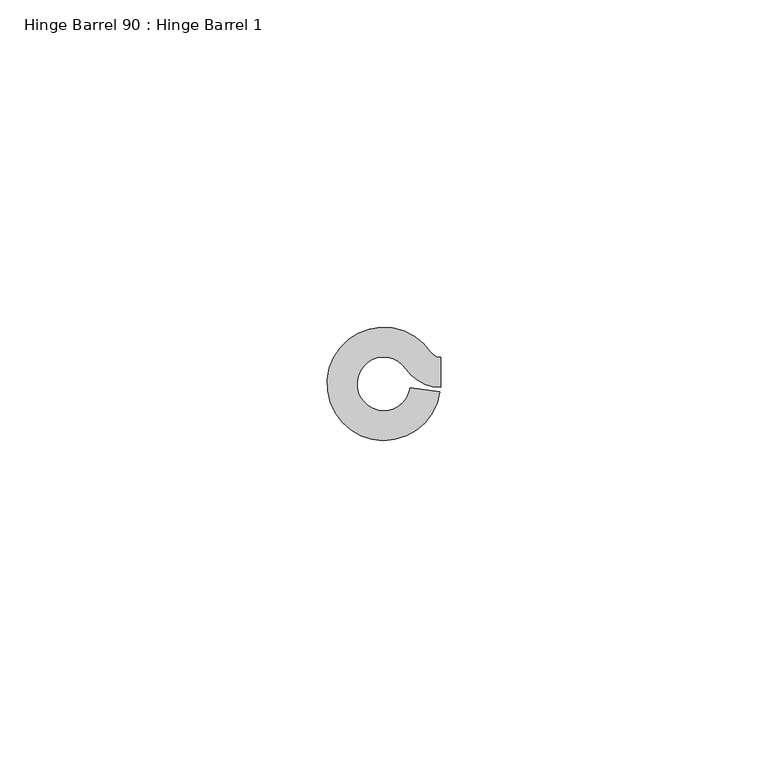
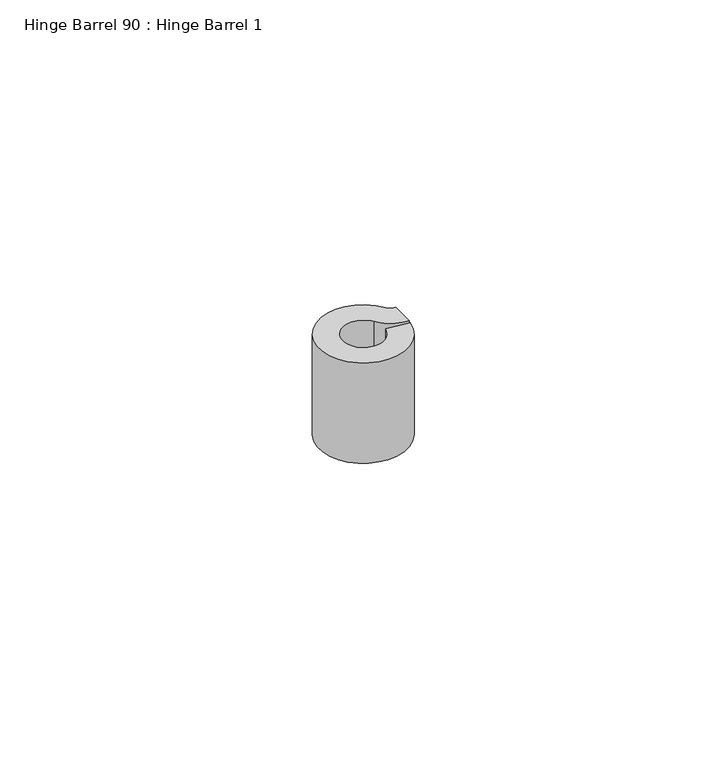
"""IFC4 building model written with IfcOpenShell, lengths in millimetres: proxy geometry, Hinge Barrel 90 : Hinge Barrel 1."""

from ifc_helpers import new_model, si_unit, point, frame, frame_2d, origin, place, context, project, spatial, polyline, circle_curve, trimmed, segment, composite_curve, outline, extrude, source, transform, mapped, element, save


def hinge_barrel_90_hinge_barrel_1_18e6ea9c(model_context):
    return source(origin(), model_context, "Body", "SweptSolid", [
        extrude(outline(composite_curve([segment(trimmed(circle_curve(frame_2d((587319.1320739, -531776.6049841)), 4.0894), [point((587322.5194669, -531774.3139665))], [point((587323.1821338, -531777.1708529))], True, "CARTESIAN"), True, "CONTINUOUS"), segment(polyline([(587323.1821338, -531777.1708529), (587327.7022899, -531777.8024028)]), True, "CONTINUOUS"), segment(trimmed(circle_curve(frame_2d((587319.1320739, -531776.6049841)), 8.6534625), [point((587327.7022899, -531777.8024028))], [point((587326.3000393, -531771.7570273))], False, "CARTESIAN"), True, "CONTINUOUS"), segment(trimmed(circle_curve(frame_2d((587327.8245257, -531770.7259615)), 1.8404226), [point((587326.3000393, -531771.7570273))], [point((587327.8245257, -531772.5663841))], True, "CARTESIAN"), True, "CONTINUOUS"), segment(polyline([(587327.8245257, -531772.5663841), (587327.8245257, -531777.1304466)]), True, "CONTINUOUS"), segment(trimmed(circle_curve(frame_2d((587327.8245257, -531770.7259615)), 6.4044851), [point((587327.8245257, -531777.1304466))], [point((587322.5194669, -531774.3139665))], False, "CARTESIAN"), True, "CONTINUOUS")], self_intersect=False)), frame((0.0, 0.0, 1250.95), z_axis=(0.0, 0.0, 1.0), x_axis=(1.0, 0.0, 0.0)), (0.0, 0.0, 1.0), 20.8359375),
    ])


if __name__ == "__main__":
    model = new_model("IFC4")
    model_context = context("Model", 3, world=origin())
    ifc_project = project(units=[si_unit("LENGTHUNIT", "METRE", prefix="MILLI")], contexts=[model_context])
    site = spatial("IfcSite", under=ifc_project)
    building = spatial("IfcBuilding", under=site)
    placement = place(None, origin())
    hinge_barrel_90_hinge_barrel_1_shape = hinge_barrel_90_hinge_barrel_1_18e6ea9c(model_context)
    element("IfcBuildingElementProxy", 1, Name="Hinge Barrel 90 : Hinge Barrel 1", ObjectType="Hinge Barrel 90 : Hinge Barrel 1", at=placement, inside=building, context=model_context, shape_type="MappedRepresentation", body=[
        mapped(hinge_barrel_90_hinge_barrel_1_shape, transform((0.0, 0.0, 0.0), x_axis=(1.0, 0.0, 0.0), y_axis=(0.0, 1.0, 0.0), z_axis=(0.0, 0.0, 1.0))),
    ])
    save(model, "model.ifc")

# Revit data of these elements
# Element 1 (IfcBuildingElementProxy, "Hinge Barrel 90 : Hinge Barrel 1")
#   Materials on its faces: "6\"X6\" WELD-ON STL BUTT HINGE"
# Materials
#   "6\"X6\" WELD-ON STL BUTT HINGE": class "Metal", colour RGB 189 187 185, transparency 0, Description = "Carbon steel", Cost = 0
